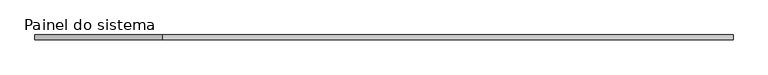
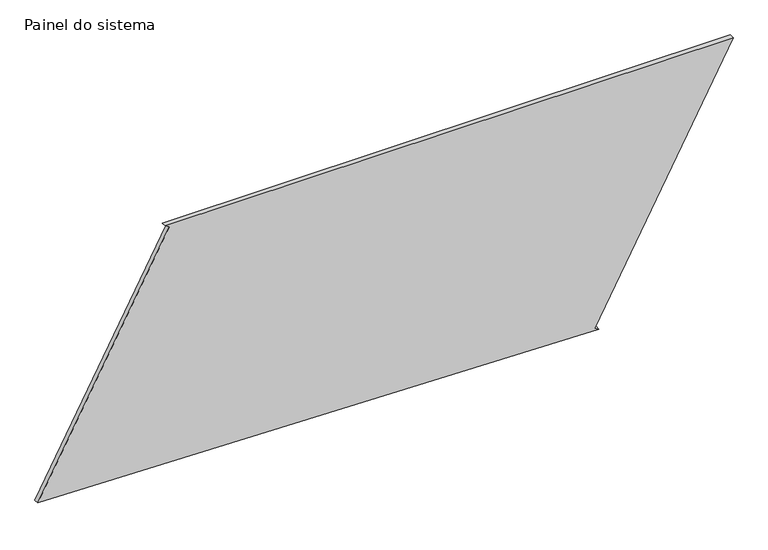
"""IFC4 building model written with IfcOpenShell, lengths in millimetres: plate geometry, Painel do sistema : Envidraçado."""

from ifc_helpers import new_model, si_unit, frame, origin, place, context, project, spatial, polyline, outline, extrude, source, transform, mapped, element, save


def painel_do_sistema_51b26320(model_context):
    return source(origin(), model_context, "Body", "SweptSolid", [
        extrude(outline(polyline([(0.0, 1086.1960663), (11.7958757, 1064.153895), (1328.0812399, 1768.5644656), (1328.0812399, -1120.9296078), (1316.2853643, -1098.8874365), (64.9042677, -1768.5644656), (0.0, 1086.1960663)])), frame((0.0, 24.5, 0.0), z_axis=(0.0, 1.0, 0.0), x_axis=(0.0, 0.0, 1.0)), (0.0, 0.0, 1.0), 25.0),
    ])


if __name__ == "__main__":
    model = new_model("IFC4")
    model_context = context("Model", 3, world=origin())
    ifc_project = project(units=[si_unit("LENGTHUNIT", "METRE", prefix="MILLI")], contexts=[model_context])
    site = spatial("IfcSite", under=ifc_project)
    building = spatial("IfcBuilding", under=site)
    placement = place(None, origin())
    painel_do_sistema_shape = painel_do_sistema_51b26320(model_context)
    element("IfcPlate", 1, ObjectType="Painel do sistema : Envidraçado", at=placement, inside=building, context=model_context, shape_type="MappedRepresentation", body=[
        mapped(painel_do_sistema_shape, transform((0.0, 0.0, 0.0), x_axis=(1.0, 0.0, 0.0), y_axis=(0.0, 1.0, 0.0), z_axis=(0.0, 0.0, 1.0))),
    ])
    save(model, "model.ifc")

# Revit data of these elements
# Type "Painel do sistema : Envidraçado"
#   Construction Type Id = "GSP4R"
#   Analytic Construction = "Vidraça única Pilkington 1/8 pol"
#   Visual Light Transmittance = 0.9
#   Solar Heat Gain Coefficient = 0.86
#   Heat Transfer Coefficient (U) = 6.7069 W/(m²·K)
# Element 1 (IfcPlate, "Painel do sistema : Envidraçado")
#   Materials on its faces: "Vidro"
# Materials
#   "Vidro": class "Vidro", colour RGB 0 128 192, transparency 0.9, Description = "Vidro de sílica", Cost = 0
